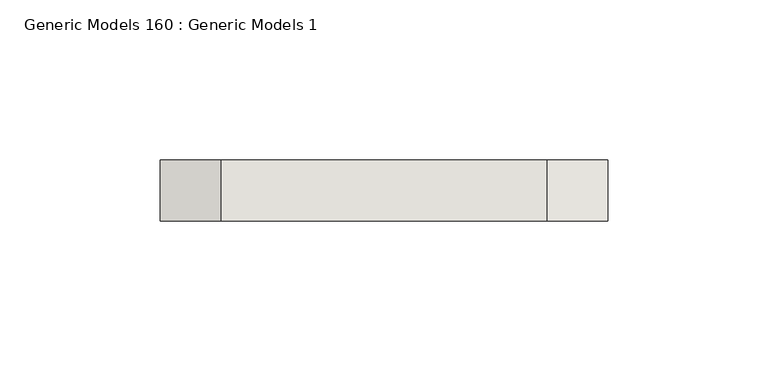
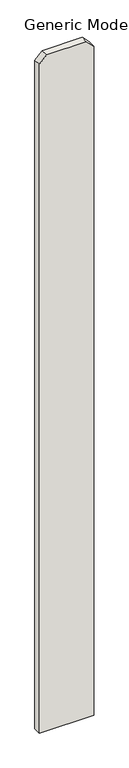
"""IFC4 building model written with IfcOpenShell, lengths in millimetres: wall geometry, Generic Models 160 : Generic Models 1."""

from ifc_helpers import new_model, si_unit, frame, origin, place, context, project, spatial, polyline, outline, extrude, source, transform, mapped, element, save


def generic_models_160_generic_models_1_6da41685(model_context):
    return source(origin(), model_context, "Body", "SweptSolid", [
        extrude(outline(polyline([(76.2, 323365.8125), (1885.95, 323365.8125), (1905.0, 323346.7625), (1905.0, 323245.1625), (1885.95, 323226.1125), (76.2, 323226.1125), (76.2, 323365.8125)])), frame((0.0, 547.6875, 0.0), z_axis=(0.0, 1.0, 0.0), x_axis=(0.0, 0.0, 1.0)), (0.0, 0.0, 1.0), 19.05),
    ])


if __name__ == "__main__":
    model = new_model("IFC4")
    model_context = context("Model", 3, world=origin())
    ifc_project = project(units=[si_unit("LENGTHUNIT", "METRE", prefix="MILLI")], contexts=[model_context])
    site = spatial("IfcSite", under=ifc_project)
    building = spatial("IfcBuilding", under=site)
    placement = place(None, origin())
    generic_models_160_generic_models_1_shape = generic_models_160_generic_models_1_6da41685(model_context)
    element("IfcWall", 1, ObjectType="Generic Models 160 : Generic Models 1", at=placement, inside=building, context=model_context, shape_type="MappedRepresentation", body=[
        mapped(generic_models_160_generic_models_1_shape, transform((0.0, 0.0, 0.0), x_axis=(1.0, 0.0, 0.0), y_axis=(0.0, 1.0, 0.0), z_axis=(0.0, 0.0, 1.0))),
    ])
    save(model, "model.ifc")

# Revit data of these elements
# Element 1 (IfcWall, "Generic Models 160 : Generic Models 1")
#   Materials on its faces: "VERTICAL 1X6 CEDAR PLANKS W/ CLEAR WOOD SEALER"
# Materials
#   "VERTICAL 1X6 CEDAR PLANKS W/ CLEAR WOOD SEALER": class "Wood", colour RGB 234 198 147, transparency 0, Description = "Pinus Echinata", Cost = 0
